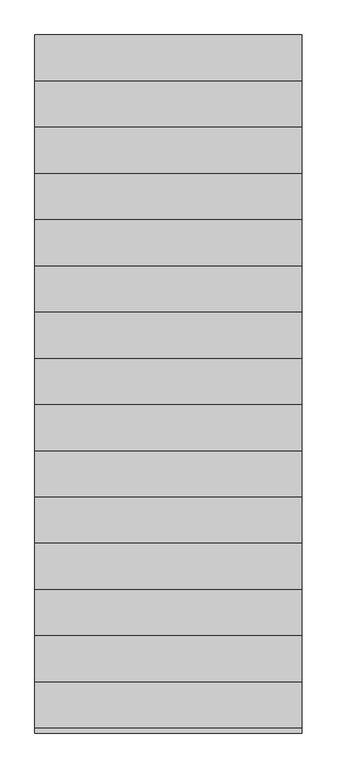
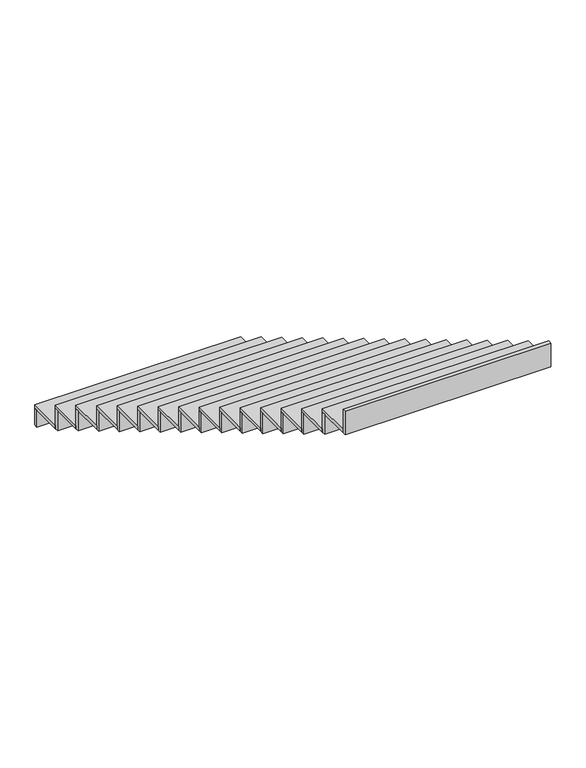
"""IFC4 building model written with IfcOpenShell, lengths in millimetres: stair flight geometry."""

from ifc_helpers import new_model, si_unit, frame, origin, place, context, project, spatial, polyline, outline, extrude, source, transform, mapped, element, save


def stair_flight_12b22758(model_context):
    return source(origin(), model_context, "Body", "SweptSolid", [
        extrude(outline(polyline([(52915.0, -1730.0), (52915.0, -1700.0), (54650.0, -1700.0), (54650.0, -1730.0), (52915.0, -1730.0)])), frame((0.0, 0.0, 7730.0), z_axis=(0.0, 0.0, 1.0), x_axis=(1.0, 0.0, 0.0)), (0.0, 0.0, 1.0), 149.375),
        extrude(outline(polyline([(54650.0, -2000.0), (52915.0, -2000.0), (52915.0, -1700.0), (54650.0, -1700.0), (54650.0, -2000.0)])), frame((0.0, 0.0, 7879.375), z_axis=(0.0, 0.0, 1.0), x_axis=(1.0, 0.0, 0.0)), (0.0, 0.0, 1.0), 30.0),
        extrude(outline(polyline([(52915.0, -2030.0), (52915.0, -2000.0), (54650.0, -2000.0), (54650.0, -2030.0), (52915.0, -2030.0)])), frame((0.0, 0.0, 7879.375), z_axis=(0.0, 0.0, 1.0), x_axis=(1.0, 0.0, 0.0)), (0.0, 0.0, 1.0), 179.375),
        extrude(outline(polyline([(54650.0, -2300.0), (52915.0, -2300.0), (52915.0, -2000.0), (54650.0, -2000.0), (54650.0, -2300.0)])), frame((0.0, 0.0, 8058.75), z_axis=(0.0, 0.0, 1.0), x_axis=(1.0, 0.0, 0.0)), (0.0, 0.0, 1.0), 30.0),
        extrude(outline(polyline([(52915.0, -2330.0), (52915.0, -2300.0), (54650.0, -2300.0), (54650.0, -2330.0), (52915.0, -2330.0)])), frame((0.0, 0.0, 8058.75), z_axis=(0.0, 0.0, 1.0), x_axis=(1.0, 0.0, 0.0)), (0.0, 0.0, 1.0), 179.375),
        extrude(outline(polyline([(54650.0, -2600.0), (52915.0, -2600.0), (52915.0, -2300.0), (54650.0, -2300.0), (54650.0, -2600.0)])), frame((0.0, 0.0, 8238.125), z_axis=(0.0, 0.0, 1.0), x_axis=(1.0, 0.0, 0.0)), (0.0, 0.0, 1.0), 30.0),
        extrude(outline(polyline([(52915.0, -2630.0), (52915.0, -2600.0), (54650.0, -2600.0), (54650.0, -2630.0), (52915.0, -2630.0)])), frame((0.0, 0.0, 8238.125), z_axis=(0.0, 0.0, 1.0), x_axis=(1.0, 0.0, 0.0)), (0.0, 0.0, 1.0), 179.375),
        extrude(outline(polyline([(54650.0, -2900.0), (52915.0, -2900.0), (52915.0, -2600.0), (54650.0, -2600.0), (54650.0, -2900.0)])), frame((0.0, 0.0, 8417.5), z_axis=(0.0, 0.0, 1.0), x_axis=(1.0, 0.0, 0.0)), (0.0, 0.0, 1.0), 30.0),
        extrude(outline(polyline([(52915.0, -2930.0), (52915.0, -2900.0), (54650.0, -2900.0), (54650.0, -2930.0), (52915.0, -2930.0)])), frame((0.0, 0.0, 8417.5), z_axis=(0.0, 0.0, 1.0), x_axis=(1.0, 0.0, 0.0)), (0.0, 0.0, 1.0), 179.375),
        extrude(outline(polyline([(54650.0, -3200.0), (52915.0, -3200.0), (52915.0, -2900.0), (54650.0, -2900.0), (54650.0, -3200.0)])), frame((0.0, 0.0, 8596.875), z_axis=(0.0, 0.0, 1.0), x_axis=(1.0, 0.0, 0.0)), (0.0, 0.0, 1.0), 30.0),
        extrude(outline(polyline([(52915.0, -3230.0), (52915.0, -3200.0), (54650.0, -3200.0), (54650.0, -3230.0), (52915.0, -3230.0)])), frame((0.0, 0.0, 8596.875), z_axis=(0.0, 0.0, 1.0), x_axis=(1.0, 0.0, 0.0)), (0.0, 0.0, 1.0), 179.375),
        extrude(outline(polyline([(54650.0, -3500.0), (52915.0, -3500.0), (52915.0, -3200.0), (54650.0, -3200.0), (54650.0, -3500.0)])), frame((0.0, 0.0, 8776.25), z_axis=(0.0, 0.0, 1.0), x_axis=(1.0, 0.0, 0.0)), (0.0, 0.0, 1.0), 30.0),
        extrude(outline(polyline([(52915.0, -3530.0), (52915.0, -3500.0), (54650.0, -3500.0), (54650.0, -3530.0), (52915.0, -3530.0)])), frame((0.0, 0.0, 8776.25), z_axis=(0.0, 0.0, 1.0), x_axis=(1.0, 0.0, 0.0)), (0.0, 0.0, 1.0), 179.375),
        extrude(outline(polyline([(54650.0, -3800.0), (52915.0, -3800.0), (52915.0, -3500.0), (54650.0, -3500.0), (54650.0, -3800.0)])), frame((0.0, 0.0, 8955.625), z_axis=(0.0, 0.0, 1.0), x_axis=(1.0, 0.0, 0.0)), (0.0, 0.0, 1.0), 30.0),
        extrude(outline(polyline([(52915.0, -3830.0), (52915.0, -3800.0), (54650.0, -3800.0), (54650.0, -3830.0), (52915.0, -3830.0)])), frame((0.0, 0.0, 8955.625), z_axis=(0.0, 0.0, 1.0), x_axis=(1.0, 0.0, 0.0)), (0.0, 0.0, 1.0), 179.375),
        extrude(outline(polyline([(54650.0, -4100.0), (52915.0, -4100.0), (52915.0, -3800.0), (54650.0, -3800.0), (54650.0, -4100.0)])), frame((0.0, 0.0, 9135.0), z_axis=(0.0, 0.0, 1.0), x_axis=(1.0, 0.0, 0.0)), (0.0, 0.0, 1.0), 30.0),
        extrude(outline(polyline([(52915.0, -4130.0), (52915.0, -4100.0), (54650.0, -4100.0), (54650.0, -4130.0), (52915.0, -4130.0)])), frame((0.0, 0.0, 9135.0), z_axis=(0.0, 0.0, 1.0), x_axis=(1.0, 0.0, 0.0)), (0.0, 0.0, 1.0), 179.375),
        extrude(outline(polyline([(54650.0, -4400.0), (52915.0, -4400.0), (52915.0, -4100.0), (54650.0, -4100.0), (54650.0, -4400.0)])), frame((0.0, 0.0, 9314.375), z_axis=(0.0, 0.0, 1.0), x_axis=(1.0, 0.0, 0.0)), (0.0, 0.0, 1.0), 30.0),
        extrude(outline(polyline([(52915.0, -4430.0), (52915.0, -4400.0), (54650.0, -4400.0), (54650.0, -4430.0), (52915.0, -4430.0)])), frame((0.0, 0.0, 9314.375), z_axis=(0.0, 0.0, 1.0), x_axis=(1.0, 0.0, 0.0)), (0.0, 0.0, 1.0), 179.375),
        extrude(outline(polyline([(54650.0, -4700.0), (52915.0, -4700.0), (52915.0, -4400.0), (54650.0, -4400.0), (54650.0, -4700.0)])), frame((0.0, 0.0, 9493.75), z_axis=(0.0, 0.0, 1.0), x_axis=(1.0, 0.0, 0.0)), (0.0, 0.0, 1.0), 30.0),
        extrude(outline(polyline([(52915.0, -4730.0), (52915.0, -4700.0), (54650.0, -4700.0), (54650.0, -4730.0), (52915.0, -4730.0)])), frame((0.0, 0.0, 9493.75), z_axis=(0.0, 0.0, 1.0), x_axis=(1.0, 0.0, 0.0)), (0.0, 0.0, 1.0), 179.375),
        extrude(outline(polyline([(54650.0, -5000.0), (52915.0, -5000.0), (52915.0, -4700.0), (54650.0, -4700.0), (54650.0, -5000.0)])), frame((0.0, 0.0, 9673.125), z_axis=(0.0, 0.0, 1.0), x_axis=(1.0, 0.0, 0.0)), (0.0, 0.0, 1.0), 30.0),
        extrude(outline(polyline([(52915.0, -5030.0), (52915.0, -5000.0), (54650.0, -5000.0), (54650.0, -5030.0), (52915.0, -5030.0)])), frame((0.0, 0.0, 9673.125), z_axis=(0.0, 0.0, 1.0), x_axis=(1.0, 0.0, 0.0)), (0.0, 0.0, 1.0), 179.375),
        extrude(outline(polyline([(54650.0, -5300.0), (52915.0, -5300.0), (52915.0, -5000.0), (54650.0, -5000.0), (54650.0, -5300.0)])), frame((0.0, 0.0, 9852.5), z_axis=(0.0, 0.0, 1.0), x_axis=(1.0, 0.0, 0.0)), (0.0, 0.0, 1.0), 30.0),
        extrude(outline(polyline([(52915.0, -5330.0), (52915.0, -5300.0), (54650.0, -5300.0), (54650.0, -5330.0), (52915.0, -5330.0)])), frame((0.0, 0.0, 9852.5), z_axis=(0.0, 0.0, 1.0), x_axis=(1.0, 0.0, 0.0)), (0.0, 0.0, 1.0), 179.375),
        extrude(outline(polyline([(54650.0, -5600.0), (52915.0, -5600.0), (52915.0, -5300.0), (54650.0, -5300.0), (54650.0, -5600.0)])), frame((0.0, 0.0, 10031.875), z_axis=(0.0, 0.0, 1.0), x_axis=(1.0, 0.0, 0.0)), (0.0, 0.0, 1.0), 30.0),
        extrude(outline(polyline([(52915.0, -5630.0), (52915.0, -5600.0), (54650.0, -5600.0), (54650.0, -5630.0), (52915.0, -5630.0)])), frame((0.0, 0.0, 10031.875), z_axis=(0.0, 0.0, 1.0), x_axis=(1.0, 0.0, 0.0)), (0.0, 0.0, 1.0), 179.375),
        extrude(outline(polyline([(54650.0, -5900.0), (52915.0, -5900.0), (52915.0, -5600.0), (54650.0, -5600.0), (54650.0, -5900.0)])), frame((0.0, 0.0, 10211.25), z_axis=(0.0, 0.0, 1.0), x_axis=(1.0, 0.0, 0.0)), (0.0, 0.0, 1.0), 30.0),
        extrude(outline(polyline([(52915.0, -5930.0), (52915.0, -5900.0), (54650.0, -5900.0), (54650.0, -5930.0), (52915.0, -5930.0)])), frame((0.0, 0.0, 10211.25), z_axis=(0.0, 0.0, 1.0), x_axis=(1.0, 0.0, 0.0)), (0.0, 0.0, 1.0), 179.375),
        extrude(outline(polyline([(52915.0, -6230.0), (52915.0, -6200.0), (54650.0, -6200.0), (54650.0, -6230.0), (52915.0, -6230.0)])), frame((0.0, 0.0, 10390.625), z_axis=(0.0, 0.0, 1.0), x_axis=(1.0, 0.0, 0.0)), (0.0, 0.0, 1.0), 209.375),
        extrude(outline(polyline([(54650.0, -6200.0), (52915.0, -6200.0), (52915.0, -5900.0), (54650.0, -5900.0), (54650.0, -6200.0)])), frame((0.0, 0.0, 10390.625), z_axis=(0.0, 0.0, 1.0), x_axis=(1.0, 0.0, 0.0)), (0.0, 0.0, 1.0), 30.0),
    ])


if __name__ == "__main__":
    model = new_model("IFC4")
    model_context = context("Model", 3, world=origin())
    ifc_project = project(units=[si_unit("LENGTHUNIT", "METRE", prefix="MILLI")], contexts=[model_context])
    site = spatial("IfcSite", under=ifc_project)
    building = spatial("IfcBuilding", under=site)
    placement = place(None, origin())
    stair_flight_shape = stair_flight_12b22758(model_context)
    element("IfcStairFlight", 1, at=placement, inside=building, context=model_context, shape_type="MappedRepresentation", body=[
        mapped(stair_flight_shape, transform((0.0, 0.0, 0.0), x_axis=(1.0, 0.0, 0.0), y_axis=(0.0, 1.0, 0.0), z_axis=(0.0, 0.0, 1.0))),
    ])
    save(model, "model.ifc")

# Revit data of these elements
# Element 1 (IfcStairFlight)
#   Materials on its faces: "00_Finish_Deco Tile"
# Materials
#   "00_Finish_Deco Tile": class "Finish", colour RGB 245 245 245, transparency 0, Description = "Ceramic Tile", Cost = 0
